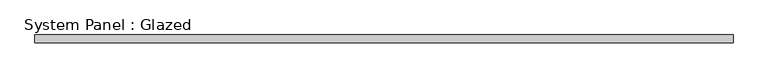
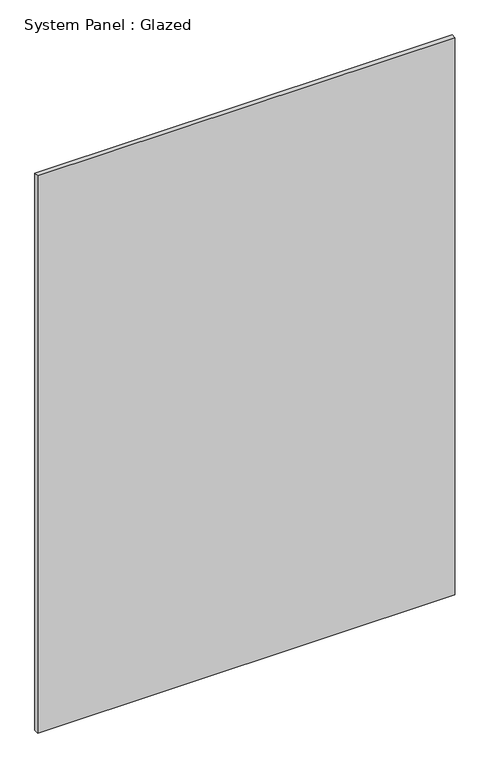
"""IFC4 building model written with IfcOpenShell, lengths in millimetres: plate geometry, System Panel : Glazed."""

from ifc_helpers import new_model, si_unit, origin, origin_with_axes, place, context, project, spatial, polyline, outline, extrude, source, transform, mapped, element, save


def system_panel_glazed_19379390(model_context):
    return source(origin(), model_context, "Body", "SweptSolid", [
        extrude(outline(polyline([(1122.415207, 24.5), (-1122.415207, 24.5), (-1122.415207, 49.5), (1122.415207, 49.5), (1122.415207, 24.5)])), origin_with_axes(), (0.0, 0.0, 1.0), 3170.0),
    ])


if __name__ == "__main__":
    model = new_model("IFC4")
    model_context = context("Model", 3, world=origin())
    ifc_project = project(units=[si_unit("LENGTHUNIT", "METRE", prefix="MILLI")], contexts=[model_context])
    site = spatial("IfcSite", under=ifc_project)
    building = spatial("IfcBuilding", under=site)
    placement = place(None, origin())
    system_panel_glazed_shape = system_panel_glazed_19379390(model_context)
    element("IfcPlate", 1, ObjectType="System Panel : Glazed", at=placement, inside=building, context=model_context, shape_type="MappedRepresentation", body=[
        mapped(system_panel_glazed_shape, transform((0.0, 0.0, 0.0), x_axis=(1.0, 0.0, 0.0), y_axis=(0.0, 1.0, 0.0), z_axis=(0.0, 0.0, 1.0))),
    ])
    save(model, "model.ifc")

# Revit data of these elements
# Type "System Panel : Glazed"
#   Construction Type Id = "GSP4R"
#   Analytic Construction = "1/8 in Pilkington single glazing"
#   Visual Light Transmittance = 0.9
#   Solar Heat Gain Coefficient = 0.86
#   Heat Transfer Coefficient (U) = 6.7069 W/(m²·K)
#   Define Thermal Properties by = 1
# Element 1 (IfcPlate, "System Panel : Glazed")
#   Materials on its faces: "Glass"
# Materials
#   "Glass": class "Glass", colour RGB 245 245 243, transparency 1, Description = "Soda Lime Glass", Cost = 0
